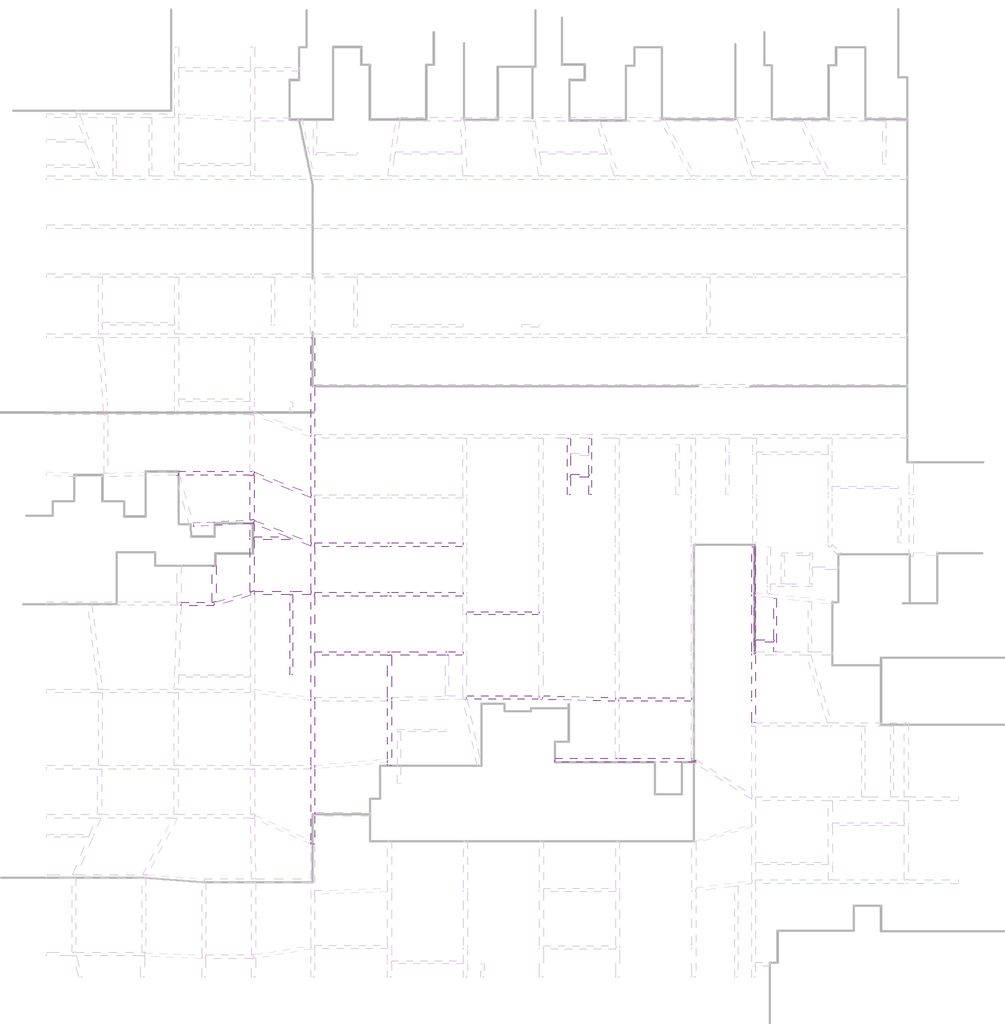
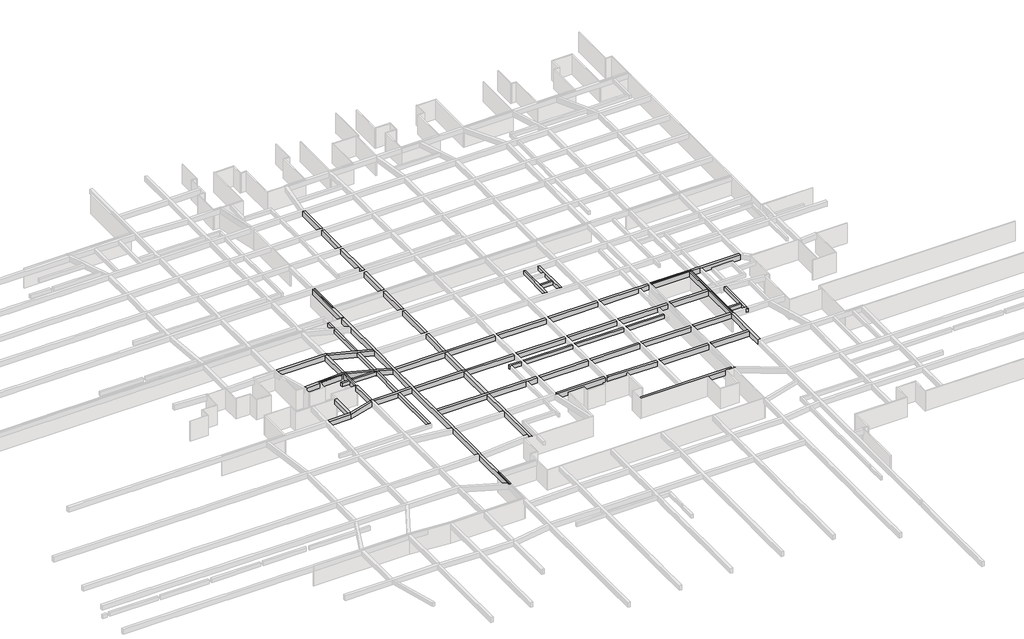
# One storey, part 13 of 16: 28 beams.
"""IFC4 building model written with IfcOpenShell, lengths in millimetres."""

from ifc_helpers import new_model, si_unit, frame, origin, place, context, project, spatial, polyline, outline, extrude, faceted_brep, element, save

model = new_model("IFC4")

# Units and contexts
model_context = context("Model", 3, world=origin())
ifc_project = project(units=[si_unit("LENGTHUNIT", "METRE", prefix="MILLI")], contexts=[model_context])

# Site, building, storey
site = spatial("IfcSite", under=ifc_project)
building = spatial("IfcBuilding", under=site)
storey = spatial("IfcBuildingStorey", under=building, Name="户型图", Elevation=0.0)

# Beams
placement = place(None, origin())
element("IfcBeam", 1, ObjectType="混凝土 - 矩形梁 : KL_beam", at=placement, inside=storey, context=model_context, shape_type="Brep", body=[
    faceted_brep([(127216.2109037, 158915.0633975, 3300.0), (127216.2109037, 158520.1276342, 3300.0), (127018.7754912, 158515.0633975, 3300.0), (127281.619868, 158515.0633975, 3300.0), (134828.9386535, 158515.0633975, 3300.0), (135228.9386535, 158515.0633975, 3300.0), (135228.9386535, 158852.5195892, 3300.0), (135228.9386535, 158915.0633975, 3300.0), (134828.9386535, 158915.0633975, 3300.0), (127018.7754912, 158515.0633975, 2500.0), (127281.619868, 158515.0633975, 2500.0), (134828.9386535, 158515.0633975, 2500.0), (135228.9386535, 158515.0633975, 2500.0), (127216.2109037, 158520.1276342, 2500.0), (127216.2109037, 158915.0633975, 2500.0), (134828.9386535, 158915.0633975, 2500.0), (135228.9386535, 158915.0633975, 2500.0), (135228.9386535, 158852.5195892, 2500.0)], [[[0, 1, 2, 3, 4, 5, 6, 7, 8]], [[2, 9, 10, 11, 12, 5, 4, 3]], [[13, 14, 15, 16, 17, 12, 11, 10, 9]], [[14, 0, 8, 7, 16, 15]], [[13, 1, 0, 14]], [[1, 13, 9, 2]], [[7, 6, 5, 12, 17, 16]]]),
])
element("IfcBeam", 2, ObjectType="混凝土 - 矩形梁 : KL_beam", at=placement, inside=storey, context=model_context, shape_type="Brep", body=[
    faceted_brep([(135228.9386535, 153383.6684969, 3300.0), (135228.9386535, 153710.917602, 3300.0), (135228.9386535, 153784.2174353, 3300.0), (134828.9386535, 153763.2543236, 3300.0), (128735.7458004, 153443.9236175, 3300.0), (128848.9009007, 153049.3048866, 3300.0), (134828.9386535, 153362.7053852, 3300.0), (134996.9527927, 153371.5106331, 3300.0), (135228.9386535, 153383.6684969, 2500.0), (128848.9009007, 153049.3048866, 2500.0), (134828.9386535, 153362.7053852, 2500.0), (134996.9527927, 153371.5106331, 2500.0), (135228.9386535, 153784.2174353, 2500.0), (135228.9386535, 153710.917602, 2500.0), (128735.7458004, 153443.9236175, 2500.0), (134828.9386535, 153763.2543236, 2500.0)], [[[0, 1, 2, 3, 4, 5, 6, 7]], [[8, 0, 7, 6, 5, 9, 10, 11]], [[12, 13, 8, 11, 10, 9, 14, 15]], [[2, 12, 15, 14, 4, 3]], [[5, 4, 14, 9]], [[2, 1, 0, 8, 13, 12]]]),
])
element("IfcBeam", 3, ObjectType="混凝土 - 矩形梁 : KL_beam", at=placement, inside=storey, context=model_context, shape_type="Brep", body=[
    faceted_brep([(135228.9386535, 158515.0633975, 3300.0), (134828.9386535, 158515.0633975, 3300.0), (134828.9386535, 153763.2543236, 3300.0), (135228.9386535, 153784.2174353, 3300.0), (135228.9386535, 158424.0615917, 3300.0), (134828.9386535, 158515.0633975, 2500.0), (134828.9386535, 153763.2543236, 2500.0), (135228.9386535, 158515.0633975, 2500.0), (135228.9386535, 158424.0615917, 2500.0), (135228.9386535, 153784.2174353, 2500.0)], [[[0, 1, 2, 3, 4]], [[1, 5, 6, 2]], [[5, 7, 8, 9, 6]], [[7, 0, 4, 3, 9, 8]], [[1, 0, 7, 5]], [[3, 2, 6, 9]]]),
])
element("IfcBeam", 4, ObjectType="混凝土 - 矩形梁 : KL_beam", at=placement, inside=storey, context=model_context, shape_type="Brep", body=[
    faceted_brep([(135228.9386535, 158852.5195892, 3300.0), (135228.9386535, 158515.0633975, 3300.0), (135228.9386535, 158424.0615917, 3300.0), (139049.0511844, 156957.6577813, 3300.0), (139349.0511844, 156842.4985708, 3300.0), (141266.2091209, 156106.5705895, 3300.0), (141266.2091209, 156535.028587, 3300.0), (139349.0511844, 157270.9565683, 3300.0), (139049.0511844, 157386.1157788, 3300.0), (135228.9386535, 158424.0615917, 2500.0), (141266.2091209, 156106.5705895, 2500.0), (135228.9386535, 158515.0633975, 2500.0), (135228.9386535, 158852.5195892, 2500.0), (141266.2091209, 156535.028587, 2500.0)], [[[0, 1, 2, 3, 4, 5, 6, 7, 8]], [[2, 9, 10, 5, 4, 3]], [[9, 11, 12, 13, 10]], [[12, 0, 8, 7, 6, 13]], [[0, 12, 11, 9, 2, 1]], [[6, 5, 10, 13]]]),
])
element("IfcBeam", 5, ObjectType="混凝土 - 矩形梁 : KL_beam", at=placement, inside=storey, context=model_context, shape_type="Brep", body=[
    faceted_brep([(135228.9386535, 153383.6684969, 3300.0), (134996.9527927, 153371.5106331, 3300.0), (135228.9386535, 153282.4596045, 3300.0), (138736.4375479, 151936.056926, 3300.0), (139049.0511844, 151816.0557941, 3300.0), (139349.0511844, 151700.8965836, 3300.0), (139517.9642674, 151636.056926, 3300.0), (141266.2091209, 150964.9686023, 3300.0), (141266.2091209, 151393.4265998, 3300.0), (139349.0511844, 152129.3545811, 3300.0), (139049.0511844, 152244.5137916, 3300.0), (135228.9386535, 153710.917602, 3300.0), (134996.9527927, 153371.5106331, 2500.0), (135228.9386535, 153282.4596045, 2500.0), (141266.2091209, 150964.9686023, 2500.0), (135228.9386535, 153383.6684969, 2500.0), (135228.9386535, 153710.917602, 2500.0), (141266.2091209, 151393.4265998, 2500.0)], [[[0, 1, 2, 3, 4, 5, 6, 7, 8, 9, 10, 11]], [[1, 12, 13, 14, 7, 6, 5, 4, 3, 2]], [[12, 15, 16, 17, 14, 13]], [[16, 11, 10, 9, 8, 17]], [[0, 15, 12, 1]], [[15, 0, 11, 16]], [[8, 7, 14, 17]]]),
])
element("IfcBeam", 6, ObjectType="混凝土 - 矩形梁 : KL_beam", at=placement, inside=storey, context=model_context, shape_type="Brep", body=[
    faceted_brep([(141266.2091209, 119283.141064, 3300.0), (141666.2091209, 119283.141064, 3300.0), (141666.2091209, 122278.0259701, 3300.0), (141666.2091209, 122678.0259701, 3300.0), (141666.2091209, 127294.7597353, 3300.0), (141666.2091209, 127696.2876703, 3300.0), (141666.2091209, 134512.5884701, 3300.0), (141666.2091209, 134912.5884701, 3300.0), (141666.2091209, 139362.5884701, 3300.0), (141666.2091209, 139762.5884701, 3300.0), (141666.2091209, 145662.5884701, 3300.0), (141666.2091209, 146062.5884701, 3300.0), (141666.2091209, 150902.424794, 3300.0), (141666.2091209, 151302.424794, 3300.0), (141666.2091209, 156044.0267812, 3300.0), (141666.2091209, 156444.0267812, 3300.0), (141666.2091209, 162447.0169772, 3300.0), (141666.2091209, 162847.0169772, 3300.0), (141666.2091209, 167762.578939, 3300.0), (141666.2091209, 168162.578939, 3300.0), (141666.2091209, 173112.5884701, 3300.0), (141266.2091209, 173112.5884701, 3300.0), (141266.2091209, 162932.5536596, 3300.0), (141266.2091209, 162504.0956621, 3300.0), (141266.2091209, 156535.028587, 3300.0), (141266.2091209, 156106.5705895, 3300.0), (141266.2091209, 151393.4265998, 3300.0), (141266.2091209, 150964.9686023, 3300.0), (141266.2091209, 146196.5023677, 3300.0), (141266.2091209, 145796.5023677, 3300.0), (141266.2091209, 134941.3479482, 3300.0), (141266.2091209, 134537.7323272, 3300.0), (141266.2091209, 127693.5189202, 3300.0), (141266.2091209, 127293.5189202, 3300.0), (141266.2091209, 119721.5942757, 3300.0), (141266.2091209, 119283.141064, 2500.0), (141266.2091209, 173112.5884701, 2500.0), (141266.2091209, 162932.5536596, 2500.0), (141266.2091209, 162504.0956621, 2500.0), (141266.2091209, 156535.028587, 2500.0), (141266.2091209, 156106.5705895, 2500.0), (141266.2091209, 151393.4265998, 2500.0), (141266.2091209, 150964.9686023, 2500.0), (141266.2091209, 146196.5023677, 2500.0), (141266.2091209, 145796.5023677, 2500.0), (141266.2091209, 134941.3479482, 2500.0), (141266.2091209, 134537.7323272, 2500.0), (141266.2091209, 127693.5189202, 2500.0), (141266.2091209, 127293.5189202, 2500.0), (141266.2091209, 119721.5942757, 2500.0), (141666.2091209, 119283.141064, 2500.0), (141666.2091209, 173112.5884701, 2500.0), (141666.2091209, 168162.578939, 2500.0), (141666.2091209, 167762.578939, 2500.0), (141666.2091209, 162847.0169772, 2500.0), (141666.2091209, 162447.0169772, 2500.0), (141666.2091209, 156444.0267812, 2500.0), (141666.2091209, 156044.0267812, 2500.0), (141666.2091209, 151302.424794, 2500.0), (141666.2091209, 150902.424794, 2500.0), (141666.2091209, 146062.5884701, 2500.0), (141666.2091209, 145662.5884701, 2500.0), (141666.2091209, 139762.5884701, 2500.0), (141666.2091209, 139362.5884701, 2500.0), (141666.2091209, 134912.5884701, 2500.0), (141666.2091209, 134512.5884701, 2500.0), (141666.2091209, 127696.2876703, 2500.0), (141666.2091209, 127294.7597353, 2500.0), (141666.2091209, 122678.0259701, 2500.0), (141666.2091209, 122278.0259701, 2500.0)], [[[0, 1, 2, 3, 4, 5, 6, 7, 8, 9, 10, 11, 12, 13, 14, 15, 16, 17, 18, 19, 20, 21, 22, 23, 24, 25, 26, 27, 28, 29, 30, 31, 32, 33, 34]], [[35, 0, 34, 33, 32, 31, 30, 29, 28, 27, 26, 25, 24, 23, 22, 21, 36, 37, 38, 39, 40, 41, 42, 43, 44, 45, 46, 47, 48, 49]], [[50, 35, 49, 48, 47, 46, 45, 44, 43, 42, 41, 40, 39, 38, 37, 36, 51, 52, 53, 54, 55, 56, 57, 58, 59, 60, 61, 62, 63, 64, 65, 66, 67, 68, 69]], [[1, 50, 69, 68, 67, 66, 65, 64, 63, 62, 61, 60, 59, 58, 57, 56, 55, 54, 53, 52, 51, 20, 19, 18, 17, 16, 15, 14, 13, 12, 11, 10, 9, 8, 7, 6, 5, 4, 3, 2]], [[21, 20, 51, 36]], [[1, 0, 35, 50]]]),
])
element("IfcBeam", 7, ObjectType="混凝土 - 矩形梁 : KL_beam", at=placement, inside=storey, context=model_context, shape_type="Brep", body=[
    faceted_brep([(141666.2091209, 151302.424794, 3300.0), (141666.2091209, 150902.424794, 3300.0), (149416.2109037, 150902.424794, 3300.0), (149816.2109037, 150902.424794, 3300.0), (157416.2109037, 150902.424794, 3300.0), (157416.2109037, 151302.424794, 3300.0), (149816.2109037, 151302.424794, 3300.0), (149416.2109037, 151302.424794, 3300.0), (141666.2091209, 150902.424794, 2500.0), (149416.2109037, 150902.424794, 2500.0), (149816.2109037, 150902.424794, 2500.0), (157416.2109037, 150902.424794, 2500.0), (141666.2091209, 151302.424794, 2500.0), (149416.2109037, 151302.424794, 2500.0), (149816.2109037, 151302.424794, 2500.0), (157416.2109037, 151302.424794, 2500.0)], [[[0, 1, 2, 3, 4, 5, 6, 7]], [[1, 8, 9, 10, 11, 4, 3, 2]], [[8, 12, 13, 14, 15, 11, 10, 9]], [[12, 0, 7, 6, 5, 15, 14, 13]], [[1, 0, 12, 8]], [[5, 4, 11, 15]]]),
    faceted_brep([(196226.5590225, 151302.424794, 3300.0), (196226.5590225, 150902.424794, 3300.0), (196226.5590225, 150902.424794, 2500.0), (196226.5590225, 151302.424794, 2500.0), (190074.1000448, 151302.424794, 3300.0), (189774.1000448, 151302.424794, 3300.0), (188616.2109037, 151302.424794, 3300.0), (188216.2109037, 151302.424794, 3300.0), (182116.2109037, 151302.424794, 3300.0), (182116.2109037, 151172.5884701, 3300.0), (188356.2109037, 151172.5884701, 3300.0), (188476.2109037, 151172.5884701, 3300.0), (188476.2109037, 150902.424794, 3300.0), (188516.2109037, 150902.424794, 3300.0), (189774.1000448, 150902.424794, 3300.0), (190074.1000448, 150902.424794, 3300.0), (188616.2109037, 151302.424794, 2500.0), (188216.2109037, 151302.424794, 2500.0), (182116.2109037, 151302.424794, 2500.0), (182116.2109037, 151172.5884701, 2500.0), (188476.2109037, 151172.5884701, 2500.0), (188476.2109037, 150902.424794, 2500.0), (188516.2109037, 150902.424794, 2500.0)], [[[0, 1, 2, 3]], [[1, 0, 4, 5, 6, 7, 8, 9, 10, 11, 12, 13, 14, 15]], [[0, 3, 16, 17, 18, 8, 7, 6, 5, 4]], [[8, 18, 19, 9]], [[12, 11, 20, 21]], [[2, 1, 15, 14, 13, 12, 21, 22]], [[20, 11, 10, 9, 19]], [[3, 2, 22, 21, 20, 19, 18, 17, 16]]]),
    faceted_brep([(157816.2109037, 150902.424794, 3300.0), (157816.2109037, 151302.424794, 3300.0), (157816.2109037, 151302.424794, 2500.0), (157816.2109037, 150902.424794, 2500.0), (165516.2109037, 151302.424794, 3300.0), (165516.2109037, 150902.424794, 3300.0), (165516.2109037, 150902.424794, 2500.0), (165516.2109037, 151302.424794, 2500.0)], [[[0, 1, 2, 3]], [[4, 5, 6, 7]], [[1, 0, 5, 4]], [[0, 3, 6, 5]], [[3, 2, 7, 6]], [[2, 1, 4, 7]]]),
    faceted_brep([(165916.2109037, 151302.424794, 3300.0), (165916.2109037, 150902.424794, 3300.0), (173616.2109037, 150902.424794, 3300.0), (173616.2109037, 151302.424794, 3300.0), (165916.2109037, 150902.424794, 2500.0), (173616.2109037, 150902.424794, 2500.0), (165916.2109037, 151302.424794, 2500.0), (173616.2109037, 151302.424794, 2500.0)], [[[0, 1, 2, 3]], [[1, 4, 5, 2]], [[4, 6, 7, 5]], [[6, 0, 3, 7]], [[1, 0, 6, 4]], [[3, 2, 5, 7]]]),
    faceted_brep([(174016.2109037, 150902.424794, 3300.0), (174016.2109037, 151302.424794, 3300.0), (174016.2109037, 151302.424794, 2500.0), (174016.2109037, 150902.424794, 2500.0), (181716.2109037, 151302.424794, 3300.0), (181716.2109037, 150902.424794, 3300.0), (181716.2109037, 150902.424794, 2500.0), (181716.2109037, 151302.424794, 2500.0), (180041.8640388, 150902.424794, 3300.0), (180341.8640388, 150902.424794, 3300.0), (180341.8640388, 151302.424794, 3300.0), (180041.8640388, 151302.424794, 3300.0)], [[[0, 1, 2, 3]], [[4, 5, 6, 7]], [[1, 0, 8, 9, 5, 4, 10, 11]], [[0, 3, 6, 5, 9, 8]], [[3, 2, 7, 6]], [[2, 1, 11, 10, 4, 7]]]),
    faceted_brep([(182116.2109037, 150902.424794, 3300.0), (182116.2109037, 150902.424794, 2500.0), (188116.2109037, 150902.424794, 2500.0), (188356.2109037, 150902.424794, 2500.0), (188356.2109037, 150902.424794, 3300.0), (188116.2109037, 150902.424794, 3300.0), (182116.2109037, 151052.5884701, 2500.0), (188356.2109037, 151052.5884701, 2500.0), (188356.2109037, 151052.5884701, 3300.0), (182116.2109037, 151052.5884701, 3300.0)], [[[0, 1, 2, 3, 4, 5]], [[3, 2, 1, 6, 7]], [[4, 3, 7, 8]], [[9, 8, 7, 6]], [[0, 5, 4, 8, 9]], [[1, 0, 9, 6]]]),
])
element("IfcBeam", 8, ObjectType="混凝土 - 矩形梁 : KL_beam", at=placement, inside=storey, context=model_context, shape_type="Brep", body=[
    faceted_brep([(141666.2091209, 146062.5884701, 3300.0), (141666.2091209, 145662.5884701, 3300.0), (149416.2109037, 145662.5884701, 3300.0), (149816.2109037, 145662.5884701, 3300.0), (157416.2109037, 145662.5884701, 3300.0), (157416.2109037, 146062.5884701, 3300.0), (149816.2109037, 146062.5884701, 3300.0), (149416.2109037, 146062.5884701, 3300.0), (141666.2091209, 145662.5884701, 2500.0), (149416.2109037, 145662.5884701, 2500.0), (149816.2109037, 145662.5884701, 2500.0), (157416.2109037, 145662.5884701, 2500.0), (141666.2091209, 146062.5884701, 2500.0), (149416.2109037, 146062.5884701, 2500.0), (149816.2109037, 146062.5884701, 2500.0), (157416.2109037, 146062.5884701, 2500.0)], [[[0, 1, 2, 3, 4, 5, 6, 7]], [[1, 8, 9, 10, 11, 4, 3, 2]], [[8, 12, 13, 14, 15, 11, 10, 9]], [[12, 0, 7, 6, 5, 15, 14, 13]], [[1, 0, 12, 8]], [[5, 4, 11, 15]]]),
    faceted_brep([(157816.2109037, 145662.5884701, 3300.0), (157816.2109037, 146062.5884701, 3300.0), (157816.2109037, 146062.5884701, 2500.0), (157816.2109037, 145662.5884701, 2500.0), (165516.2109037, 146062.5884701, 3300.0), (165516.2109037, 145662.5884701, 3300.0), (165516.2109037, 145662.5884701, 2500.0), (165516.2109037, 146062.5884701, 2500.0)], [[[0, 1, 2, 3]], [[4, 5, 6, 7]], [[1, 0, 5, 4]], [[0, 3, 6, 5]], [[3, 2, 7, 6]], [[2, 1, 4, 7]]]),
    faceted_brep([(165916.2109037, 146062.5884701, 3300.0), (165916.2109037, 145662.5884701, 3300.0), (173616.2109037, 145662.5884701, 3300.0), (173616.2109037, 146062.5884701, 3300.0), (165916.2109037, 145662.5884701, 2500.0), (173616.2109037, 145662.5884701, 2500.0), (165916.2109037, 146062.5884701, 2500.0), (173616.2109037, 146062.5884701, 2500.0)], [[[0, 1, 2, 3]], [[1, 4, 5, 2]], [[4, 6, 7, 5]], [[6, 0, 3, 7]], [[1, 0, 6, 4]], [[3, 2, 5, 7]]]),
    faceted_brep([(174016.2109037, 145662.5884701, 3300.0), (174016.2109037, 146062.5884701, 3300.0), (174016.2109037, 146062.5884701, 2500.0), (174016.2109037, 145662.5884701, 2500.0), (181716.2109037, 146062.5884701, 3300.0), (181716.2109037, 145662.5884701, 3300.0), (181716.2109037, 145662.5884701, 2500.0), (181716.2109037, 146062.5884701, 2500.0), (180041.8640388, 145662.5884701, 3300.0), (180341.8640388, 145662.5884701, 3300.0), (180341.8640388, 146062.5884701, 3300.0), (180041.8640388, 146062.5884701, 3300.0)], [[[0, 1, 2, 3]], [[4, 5, 6, 7]], [[1, 0, 8, 9, 5, 4, 10, 11]], [[0, 3, 6, 5, 9, 8]], [[3, 2, 7, 6]], [[2, 1, 11, 10, 4, 7]]]),
    faceted_brep([(182116.2109037, 145662.5884701, 3300.0), (182116.2109037, 146062.5884701, 3300.0), (182116.2109037, 146062.5884701, 2500.0), (182116.2109037, 145662.5884701, 2500.0), (188116.2109037, 145662.5884701, 3300.0), (188116.2109037, 146062.5884701, 3300.0), (188116.2109037, 145662.5884701, 2500.0), (188116.2109037, 146062.5884701, 2500.0)], [[[0, 1, 2, 3]], [[1, 0, 4, 5]], [[0, 3, 6, 4]], [[3, 2, 7, 6]], [[2, 1, 5, 7]], [[5, 4, 6, 7]]]),
])
element("IfcBeam", 9, ObjectType="混凝土 - 矩形梁 : KL_beam", at=placement, inside=storey, context=model_context, shape_type="Brep", body=[
    faceted_brep([(141666.2091209, 139762.5884701, 3300.0), (141666.2091209, 139362.5884701, 3300.0), (149416.2109037, 139362.5884701, 3300.0), (149816.2109037, 139362.5884701, 3300.0), (155575.8505966, 139362.5884701, 3300.0), (155875.8505966, 139362.5884701, 3300.0), (157416.2109037, 139362.5884701, 3300.0), (157416.2109037, 139762.5884701, 3300.0), (155875.8505966, 139762.5884701, 3300.0), (155575.8505966, 139762.5884701, 3300.0), (149816.2109037, 139762.5884701, 3300.0), (149416.2109037, 139762.5884701, 3300.0), (141666.2091209, 139362.5884701, 2500.0), (149416.2109037, 139362.5884701, 2500.0), (149816.2109037, 139362.5884701, 2500.0), (157416.2109037, 139362.5884701, 2500.0), (141666.2091209, 139762.5884701, 2500.0), (149416.2109037, 139762.5884701, 2500.0), (149816.2109037, 139762.5884701, 2500.0), (157416.2109037, 139762.5884701, 2500.0)], [[[0, 1, 2, 3, 4, 5, 6, 7, 8, 9, 10, 11]], [[1, 12, 13, 14, 15, 6, 5, 4, 3, 2]], [[12, 16, 17, 18, 19, 15, 14, 13]], [[16, 0, 11, 10, 9, 8, 7, 19, 18, 17]], [[1, 0, 16, 12]], [[7, 6, 15, 19]]]),
    faceted_brep([(157816.2109037, 139362.5884701, 3300.0), (157816.2109037, 139762.5884701, 3300.0), (157816.2109037, 139762.5884701, 2500.0), (157816.2109037, 139362.5884701, 2500.0), (165516.2109037, 139762.5884701, 3300.0), (165516.2109037, 139362.5884701, 3300.0), (165516.2109037, 139362.5884701, 2500.0), (165516.2109037, 139762.5884701, 2500.0)], [[[0, 1, 2, 3]], [[4, 5, 6, 7]], [[1, 0, 5, 4]], [[0, 3, 6, 5]], [[3, 2, 7, 6]], [[2, 1, 4, 7]]]),
    faceted_brep([(165916.2109037, 139762.5884701, 3300.0), (165916.2109037, 139362.5884701, 3300.0), (173616.2109037, 139362.5884701, 3300.0), (173616.2109037, 139762.5884701, 3300.0), (165916.2109037, 139362.5884701, 2500.0), (173616.2109037, 139362.5884701, 2500.0), (165916.2109037, 139762.5884701, 2500.0), (173616.2109037, 139762.5884701, 2500.0)], [[[0, 1, 2, 3]], [[1, 4, 5, 2]], [[4, 6, 7, 5]], [[6, 0, 3, 7]], [[1, 0, 6, 4]], [[3, 2, 5, 7]]]),
    faceted_brep([(174016.2109037, 139362.5884701, 3300.0), (174016.2109037, 139762.5884701, 3300.0), (174016.2109037, 139762.5884701, 2500.0), (174016.2109037, 139362.5884701, 2500.0), (181716.2109037, 139762.5884701, 3300.0), (181716.2109037, 139362.5884701, 3300.0), (181716.2109037, 139362.5884701, 2500.0), (181716.2109037, 139762.5884701, 2500.0)], [[[0, 1, 2, 3]], [[4, 5, 6, 7]], [[1, 0, 5, 4]], [[0, 3, 6, 5]], [[3, 2, 7, 6]], [[2, 1, 4, 7]]]),
    faceted_brep([(182116.2109037, 139362.5884701, 3300.0), (182116.2109037, 139762.5884701, 3300.0), (182116.2109037, 139762.5884701, 2500.0), (182116.2109037, 139362.5884701, 2500.0), (188116.2109037, 139362.5884701, 3300.0), (188116.2109037, 139762.5884701, 3300.0), (188116.2109037, 139362.5884701, 2500.0), (188116.2109037, 139762.5884701, 2500.0)], [[[0, 1, 2, 3]], [[1, 0, 4, 5]], [[0, 3, 6, 4]], [[3, 2, 7, 6]], [[2, 1, 5, 7]], [[5, 4, 6, 7]]]),
])
element("IfcBeam", 10, ObjectType="混凝土 - 矩形梁 : KL_beam", at=placement, inside=storey, context=model_context, shape_type="Brep", body=[
    faceted_brep([(157816.2109037, 135095.7397162, 3300.0), (157816.2109037, 134700.2382994, 3300.0), (157618.4857796, 134695.7397162, 3300.0), (157863.190335, 134695.7397162, 3300.0), (165516.2109037, 134695.7397162, 3300.0), (165516.2109037, 135095.7397162, 3300.0), (157618.4857796, 134695.7397162, 2500.0), (157863.190335, 134695.7397162, 2500.0), (165516.2109037, 134695.7397162, 2500.0), (157816.2109037, 134700.2382994, 2500.0), (157816.2109037, 135095.7397162, 2500.0), (165516.2109037, 135095.7397162, 2500.0)], [[[0, 1, 2, 3, 4, 5]], [[2, 6, 7, 8, 4, 3]], [[9, 10, 11, 8, 7, 6]], [[10, 0, 5, 11]], [[9, 1, 0, 10]], [[1, 9, 6, 2]], [[5, 4, 8, 11]]]),
])
element("IfcBeam", 11, ObjectType="混凝土 - 矩形梁 : KL_beam", at=placement, inside=storey, context=model_context, shape_type="SweptSolid", body=[
    extrude(outline(polyline([(165916.2109037, 134695.7397162), (165916.2109037, 135090.2366531), (173616.2109037, 134875.3714487), (173616.2109037, 134475.2157459), (165713.4209895, 134695.7397162), (165916.2109037, 134695.7397162)])), frame((0.0, 0.0, 2500.0), z_axis=(0.0, 0.0, 1.0), x_axis=(1.0, 0.0, 0.0)), (0.0, 0.0, 1.0), 800.0),
])
element("IfcBeam", 12, ObjectType="混凝土 - 矩形梁 : KL_beam", at=placement, inside=storey, context=model_context, shape_type="SweptSolid", body=[
    extrude(outline(polyline([(174016.2109037, 134469.7126829), (174016.2109037, 134869.7126829), (181716.2109037, 134869.7126829), (181716.2109037, 134469.7126829), (174016.2109037, 134469.7126829)])), frame((0.0, 0.0, 2500.0), z_axis=(0.0, 0.0, 1.0), x_axis=(1.0, 0.0, 0.0)), (0.0, 0.0, 1.0), 800.0),
    extrude(outline(polyline([(182116.2109037, 134469.7126829), (182116.2109037, 134869.7126829), (188116.2109037, 134869.7126829), (188116.2109037, 134469.7126829), (182116.2109037, 134469.7126829)])), frame((0.0, 0.0, 2500.0), z_axis=(0.0, 0.0, 1.0), x_axis=(1.0, 0.0, 0.0)), (0.0, 0.0, 1.0), 800.0),
])
element("IfcBeam", 13, ObjectType="混凝土 - 矩形梁 : KL_beam", at=placement, inside=storey, context=model_context, shape_type="Brep", body=[
    faceted_brep([(167203.7499662, 128412.5884701, 3300.0), (167203.7499662, 128412.5884701, 2500.0), (167203.7499662, 128012.5884701, 2500.0), (167203.7499662, 128012.5884701, 3300.0), (182116.2109037, 128012.5884701, 3300.0), (182116.2109037, 128072.5884701, 3300.0), (182116.2109037, 128212.6640931, 3300.0), (182017.7367524, 128212.6640931, 3300.0), (182017.7367524, 128072.5884701, 3300.0), (181897.7367524, 128072.5884701, 3300.0), (181897.7367524, 128212.6640931, 3300.0), (181716.2109037, 128212.6640931, 3300.0), (181716.2109037, 128412.5884701, 3300.0), (174016.2109037, 128412.5884701, 3300.0), (173616.2109037, 128412.5884701, 3300.0), (182116.2109037, 128012.5884701, 2500.0), (173616.2109037, 128412.5884701, 2500.0), (174016.2109037, 128412.5884701, 2500.0), (181716.2109037, 128412.5884701, 2500.0), (181716.2109037, 128212.6640931, 2500.0), (181897.7367524, 128212.6640931, 2500.0), (181897.7367524, 128072.5884701, 2500.0), (182017.7367524, 128072.5884701, 2500.0), (182017.7367524, 128212.6640931, 2500.0), (182116.2109037, 128212.6640931, 2500.0), (182116.2109037, 128072.5884701, 2500.0)], [[[0, 1, 2, 3]], [[0, 3, 4, 5, 6, 7, 8, 9, 10, 11, 12, 13, 14]], [[3, 2, 15, 4]], [[2, 1, 16, 17, 18, 19, 20, 21, 22, 23, 24, 25, 15]], [[1, 0, 14, 13, 12, 18, 17, 16]], [[4, 15, 25, 24, 6, 5]], [[12, 11, 19, 18]], [[6, 24, 23, 7]], [[22, 8, 7, 23]], [[9, 21, 20, 10]], [[8, 22, 21, 9]], [[19, 11, 10, 20]]]),
])
element("IfcBeam", 14, ObjectType="混凝土 - 矩形梁 : KL_beam", at=placement, inside=storey, context=model_context, shape_type="Brep", body=[
    faceted_brep([(149816.2109037, 127638.3828431, 3300.0), (149416.2109037, 127638.3828431, 3300.0), (149416.2109037, 127638.3828431, 2500.0), (149816.2109037, 127638.3828431, 2500.0), (149816.2109037, 134518.224679, 3300.0), (149816.2109037, 134918.3281936, 3300.0), (149816.2109037, 139362.5884701, 3300.0), (149416.2109037, 139362.5884701, 3300.0), (149416.2109037, 134912.5884701, 3300.0), (149416.2109037, 134512.5884701, 3300.0), (149416.2109037, 128374.3249686, 3300.0), (149416.2109037, 127972.7970336, 3300.0), (149416.2109037, 139362.5884701, 2500.0), (149416.2109037, 134912.5884701, 2500.0), (149416.2109037, 134512.5884701, 2500.0), (149416.2109037, 128374.3249686, 2500.0), (149416.2109037, 127972.7970336, 2500.0), (149816.2109037, 139362.5884701, 2500.0), (149816.2109037, 134918.3281936, 2500.0), (149816.2109037, 134518.224679, 2500.0)], [[[0, 1, 2, 3]], [[1, 0, 4, 5, 6, 7, 8, 9, 10, 11]], [[2, 1, 11, 10, 9, 8, 7, 12, 13, 14, 15, 16]], [[3, 2, 16, 15, 14, 13, 12, 17, 18, 19]], [[0, 3, 19, 18, 17, 6, 5, 4]], [[7, 6, 17, 12]]]),
    faceted_brep([(149416.2109037, 189895.7397162, 3300.0), (149816.2109037, 189895.7397162, 3300.0), (149816.2109037, 189895.7397162, 2500.0), (149416.2109037, 189895.7397162, 2500.0), (149816.2109037, 185072.5884701, 3300.0), (149416.2109037, 185072.5884701, 3300.0), (149416.2109037, 185072.5884701, 2500.0), (149816.2109037, 185072.5884701, 2500.0)], [[[0, 1, 2, 3]], [[4, 5, 6, 7]], [[1, 0, 5, 4]], [[0, 3, 6, 5]], [[3, 2, 7, 6]], [[2, 1, 4, 7]]]),
    faceted_brep([(149416.2109037, 184672.5884701, 3300.0), (149816.2109037, 184672.5884701, 3300.0), (149816.2109037, 184672.5884701, 2500.0), (149416.2109037, 184672.5884701, 2500.0), (149816.2109037, 179912.5884701, 3300.0), (149416.2109037, 179912.5884701, 3300.0), (149416.2109037, 179912.5884701, 2500.0), (149816.2109037, 179912.5884701, 2500.0)], [[[0, 1, 2, 3]], [[4, 5, 6, 7]], [[1, 0, 5, 4]], [[0, 3, 6, 5]], [[3, 2, 7, 6]], [[2, 1, 4, 7]]]),
    faceted_brep([(149416.2109037, 179512.5884701, 3300.0), (149816.2109037, 179512.5884701, 3300.0), (149816.2109037, 179512.5884701, 2500.0), (149416.2109037, 179512.5884701, 2500.0), (149816.2109037, 173512.5884701, 3300.0), (149416.2109037, 173512.5884701, 3300.0), (149416.2109037, 173512.5884701, 2500.0), (149816.2109037, 173512.5884701, 2500.0), (149416.2109037, 174520.6993439, 3300.0), (149416.2109037, 174220.6993439, 3300.0), (149816.2109037, 174220.6993439, 3300.0), (149816.2109037, 174520.6993439, 3300.0)], [[[0, 1, 2, 3]], [[4, 5, 6, 7]], [[1, 0, 8, 9, 5, 4, 10, 11]], [[0, 3, 6, 5, 9, 8]], [[3, 2, 7, 6]], [[2, 1, 11, 10, 4, 7]]]),
    faceted_brep([(149416.2109037, 173112.5884701, 3300.0), (149816.2109037, 173112.5884701, 3300.0), (149816.2109037, 173112.5884701, 2500.0), (149416.2109037, 173112.5884701, 2500.0), (149816.2109037, 168162.578939, 3300.0), (149416.2109037, 168162.578939, 3300.0), (149416.2109037, 168162.578939, 2500.0), (149816.2109037, 168162.578939, 2500.0)], [[[0, 1, 2, 3]], [[4, 5, 6, 7]], [[1, 0, 5, 4]], [[0, 3, 6, 5]], [[3, 2, 7, 6]], [[2, 1, 4, 7]]]),
    faceted_brep([(149416.2109037, 162447.0169772, 3300.0), (149816.2109037, 162447.0169772, 3300.0), (149816.2109037, 162447.0169772, 2500.0), (149416.2109037, 162447.0169772, 2500.0), (149816.2109037, 156444.0267812, 3300.0), (149416.2109037, 156444.0267812, 3300.0), (149416.2109037, 156444.0267812, 2500.0), (149816.2109037, 156444.0267812, 2500.0)], [[[0, 1, 2, 3]], [[4, 5, 6, 7]], [[1, 0, 5, 4]], [[0, 3, 6, 5]], [[3, 2, 7, 6]], [[2, 1, 4, 7]]]),
    faceted_brep([(149816.2109037, 162847.0169772, 3300.0), (149416.2109037, 162847.0169772, 3300.0), (149416.2109037, 162847.0169772, 2500.0), (149816.2109037, 162847.0169772, 2500.0), (149816.2109037, 167762.578939, 3300.0), (149416.2109037, 167762.578939, 3300.0), (149416.2109037, 167762.578939, 2500.0), (149816.2109037, 167762.578939, 2500.0)], [[[0, 1, 2, 3]], [[1, 0, 4, 5]], [[2, 1, 5, 6]], [[3, 2, 6, 7]], [[0, 3, 7, 4]], [[5, 4, 7, 6]]]),
    faceted_brep([(149416.2109037, 156044.0267812, 3300.0), (149816.2109037, 156044.0267812, 3300.0), (149816.2109037, 156044.0267812, 2500.0), (149416.2109037, 156044.0267812, 2500.0), (149816.2109037, 151302.424794, 3300.0), (149416.2109037, 151302.424794, 3300.0), (149416.2109037, 151302.424794, 2500.0), (149816.2109037, 151302.424794, 2500.0)], [[[0, 1, 2, 3]], [[4, 5, 6, 7]], [[1, 0, 5, 4]], [[0, 3, 6, 5]], [[3, 2, 7, 6]], [[2, 1, 4, 7]]]),
    faceted_brep([(149416.2109037, 150902.424794, 3300.0), (149816.2109037, 150902.424794, 3300.0), (149816.2109037, 150902.424794, 2500.0), (149416.2109037, 150902.424794, 2500.0), (149816.2109037, 146062.5884701, 3300.0), (149416.2109037, 146062.5884701, 3300.0), (149416.2109037, 146062.5884701, 2500.0), (149816.2109037, 146062.5884701, 2500.0)], [[[0, 1, 2, 3]], [[4, 5, 6, 7]], [[1, 0, 5, 4]], [[0, 3, 6, 5]], [[3, 2, 7, 6]], [[2, 1, 4, 7]]]),
    faceted_brep([(149416.2109037, 145662.5884701, 3300.0), (149816.2109037, 145662.5884701, 3300.0), (149816.2109037, 145662.5884701, 2500.0), (149416.2109037, 145662.5884701, 2500.0), (149816.2109037, 139762.5884701, 3300.0), (149416.2109037, 139762.5884701, 3300.0), (149416.2109037, 139762.5884701, 2500.0), (149816.2109037, 139762.5884701, 2500.0)], [[[0, 1, 2, 3]], [[4, 5, 6, 7]], [[1, 0, 5, 4]], [[0, 3, 6, 5]], [[3, 2, 7, 6]], [[2, 1, 4, 7]]]),
])
element("IfcBeam", 15, ObjectType="混凝土 - 矩形梁 : KL_beam", at=placement, inside=storey, context=model_context, shape_type="Brep", body=[
    faceted_brep([(188116.2109037, 132211.3072201, 3300.0), (188516.2109037, 132211.3072201, 3300.0), (188516.2109037, 139362.5884701, 3300.0), (188516.2109037, 139762.5884701, 3300.0), (188516.2109037, 140731.0377403, 3300.0), (188516.2109037, 141031.0377403, 3300.0), (188516.2109037, 145641.0174941, 3300.0), (188516.2109037, 146043.11753, 3300.0), (188516.2109037, 146655.8638084, 3300.0), (188516.2109037, 146955.8638084, 3300.0), (188516.2109037, 150902.424794, 3300.0), (188476.2109037, 150902.424794, 3300.0), (188476.2109037, 139562.5884701, 3300.0), (188356.2109037, 139562.5884701, 3300.0), (188356.2109037, 150902.424794, 3300.0), (188116.2109037, 150902.424794, 3300.0), (188116.2109037, 146062.5884701, 3300.0), (188116.2109037, 145662.5884701, 3300.0), (188116.2109037, 139762.5884701, 3300.0), (188116.2109037, 139362.5884701, 3300.0), (188116.2109037, 134869.7126829, 3300.0), (188116.2109037, 134469.7126829, 3300.0), (188516.2109037, 132211.3072201, 2500.0), (188516.2109037, 139362.5884701, 2500.0), (188516.2109037, 139762.5884701, 2500.0), (188516.2109037, 145641.0174941, 2500.0), (188516.2109037, 146043.11753, 2500.0), (188516.2109037, 150902.424794, 2500.0), (188116.2109037, 132211.3072201, 2500.0), (188116.2109037, 134469.7126829, 2500.0), (188116.2109037, 134869.7126829, 2500.0), (188116.2109037, 139362.5884701, 2500.0), (188116.2109037, 139762.5884701, 2500.0), (188116.2109037, 145662.5884701, 2500.0), (188116.2109037, 146062.5884701, 2500.0), (188116.2109037, 150902.424794, 2500.0), (188356.2109037, 150902.424794, 2500.0), (188356.2109037, 139562.5884701, 2500.0), (188476.2109037, 139562.5884701, 2500.0), (188476.2109037, 150902.424794, 2500.0)], [[[0, 1, 2, 3, 4, 5, 6, 7, 8, 9, 10, 11, 12, 13, 14, 15, 16, 17, 18, 19, 20, 21]], [[1, 22, 23, 24, 25, 26, 27, 10, 9, 8, 7, 6, 5, 4, 3, 2]], [[22, 28, 29, 30, 31, 32, 33, 34, 35, 36, 37, 38, 39, 27, 26, 25, 24, 23]], [[28, 0, 21, 20, 19, 18, 17, 16, 15, 35, 34, 33, 32, 31, 30, 29]], [[1, 0, 28, 22]], [[35, 15, 14, 36]], [[13, 37, 36, 14]], [[38, 12, 11, 39]], [[10, 27, 39, 11]], [[37, 13, 12, 38]]]),
])
element("IfcBeam", 16, ObjectType="混凝土 - 矩形梁 : KL_beam", at=placement, inside=storey, context=model_context, shape_type="Brep", body=[
    faceted_brep([(131003.4020759, 144613.3955863, 3300.0), (130946.8040559, 145013.3955863, 3300.0), (130775.1030659, 145013.3955863, 3300.0), (127482.2091287, 145013.3955863, 3300.0), (127468.2408209, 144613.3955863, 3300.0), (131003.4020759, 144613.3955863, 2500.0), (127468.2408209, 144613.3955863, 2500.0), (130946.8040559, 145013.3955863, 2500.0), (127482.2091287, 145013.3955863, 2500.0), (130775.1030659, 145013.3955863, 2500.0)], [[[0, 1, 2, 3, 4]], [[5, 0, 4, 6]], [[7, 5, 6, 8, 9]], [[1, 7, 9, 8, 3, 2]], [[4, 3, 8, 6]], [[1, 0, 5, 7]]]),
])
element("IfcBeam", 17, ObjectType="混凝土 - 矩形梁 : KL_beam", at=placement, inside=storey, context=model_context, shape_type="Brep", body=[
    faceted_brep([(134872.1367776, 146146.9200065, 3300.0), (134869.7438693, 146146.2290026, 3300.0), (134828.9386535, 146134.4456171, 3300.0), (131175.1030659, 145079.3218456, 3300.0), (130946.8040559, 145013.3955863, 3300.0), (131003.4020759, 144613.3955863, 3300.0), (134872.1367776, 145730.5761084, 3300.0), (131003.4020759, 144613.3955863, 2500.0), (134872.1367776, 145730.5761084, 2500.0), (130946.8040559, 145013.3955863, 2500.0), (131175.1030659, 145079.3218456, 2500.0), (134828.9386535, 146134.4456171, 2500.0), (134869.7438693, 146146.2290026, 2500.0), (134872.1367776, 146146.9200065, 2500.0)], [[[0, 1, 2, 3, 4, 5, 6]], [[5, 7, 8, 6]], [[9, 10, 11, 12, 13, 8, 7]], [[4, 3, 2, 1, 0, 13, 12, 11, 10, 9]], [[4, 9, 7, 5]], [[0, 6, 8, 13]]]),
])
element("IfcBeam", 18, ObjectType="混凝土 - 矩形梁 : KL_beam", at=placement, inside=storey, context=model_context, shape_type="Brep", body=[
    faceted_brep([(134872.1367776, 146146.9200065, 3300.0), (135272.1367776, 146146.9200065, 3300.0), (135272.1367776, 145846.084729, 3300.0), (135272.1367776, 145796.5023677, 3300.0), (139049.0511844, 145796.5023677, 3300.0), (139349.0511844, 145796.5023677, 3300.0), (141266.2091209, 145796.5023677, 3300.0), (141266.2091209, 146196.5023677, 3300.0), (139349.0511844, 146196.5023677, 3300.0), (139049.0511844, 146196.5023677, 3300.0), (135228.9386535, 146196.5023677, 3300.0), (134869.7438693, 146196.5023677, 3300.0), (134869.7438693, 146146.2290026, 3300.0), (135272.1367776, 145796.5023677, 2500.0), (141266.2091209, 145796.5023677, 2500.0), (135272.1367776, 146146.9200065, 2500.0), (134872.1367776, 146146.9200065, 2500.0), (134869.7438693, 146146.2290026, 2500.0), (134869.7438693, 146196.5023677, 2500.0), (135228.9386535, 146196.5023677, 2500.0), (141266.2091209, 146196.5023677, 2500.0), (135272.1367776, 145846.084729, 2500.0)], [[[0, 1, 2, 3, 4, 5, 6, 7, 8, 9, 10, 11, 12]], [[3, 13, 14, 6, 5, 4]], [[15, 16, 17, 18, 19, 20, 14, 13, 21]], [[18, 11, 10, 9, 8, 7, 20, 19]], [[11, 18, 17, 12]], [[1, 15, 21, 13, 3, 2]], [[15, 1, 0, 16]], [[16, 0, 12, 17]], [[7, 6, 14, 20]]]),
])
element("IfcBeam", 19, ObjectType="混凝土 - 矩形梁 : KL_beam", at=placement, inside=storey, context=model_context, shape_type="Brep", body=[
    faceted_brep([(134996.9527927, 153371.5106331, 3300.0), (134828.9386535, 153362.7053852, 3300.0), (134828.9386535, 151936.056926, 3300.0), (134828.9386535, 151636.056926, 3300.0), (134828.9386535, 146134.4456171, 3300.0), (134869.7438693, 146146.2290026, 3300.0), (134869.7438693, 146196.5023677, 3300.0), (135228.9386535, 146196.5023677, 3300.0), (135228.9386535, 151636.056926, 3300.0), (135228.9386535, 151936.056926, 3300.0), (135228.9386535, 153282.4596045, 3300.0), (134828.9386535, 153362.7053852, 2500.0), (134828.9386535, 146134.4456171, 2500.0), (134996.9527927, 153371.5106331, 2500.0), (135228.9386535, 153282.4596045, 2500.0), (135228.9386535, 146196.5023677, 2500.0), (134869.7438693, 146196.5023677, 2500.0), (134869.7438693, 146146.2290026, 2500.0)], [[[0, 1, 2, 3, 4, 5, 6, 7, 8, 9, 10]], [[1, 11, 12, 4, 3, 2]], [[11, 13, 14, 15, 16, 17, 12]], [[14, 10, 9, 8, 7, 15]], [[11, 1, 0, 13]], [[0, 10, 14, 13]], [[4, 12, 17, 5]], [[6, 16, 15, 7]], [[16, 6, 5, 17]]]),
])
element("IfcBeam", 20, ObjectType="混凝土 - 矩形梁 : KL_beam", at=placement, inside=storey, context=model_context, shape_type="SweptSolid", body=[
    extrude(outline(polyline([(130775.1030659, 148884.5232782), (131175.1030659, 148884.5232782), (131175.1030659, 145079.3218456), (130946.8040559, 145013.3955863), (130775.1030659, 145013.3955863), (130775.1030659, 148884.5232782)])), frame((0.0, 0.0, 2500.0), z_axis=(0.0, 0.0, 1.0), x_axis=(1.0, 0.0, 0.0)), (0.0, 0.0, 1.0), 800.0),
])
element("IfcBeam", 21, ObjectType="混凝土 - 矩形梁 : L_beam", at=placement, inside=storey, context=model_context, shape_type="Brep", body=[
    faceted_brep([(168841.2109037, 162447.0169772, 3300.0), (168541.2109037, 162447.0169772, 3300.0), (168541.2109037, 156444.0267812, 3300.0), (168841.2109037, 156444.0267812, 3300.0), (168841.2109037, 158287.5884701, 3300.0), (168841.2109037, 158587.5884701, 3300.0), (168841.2109037, 160537.5884701, 3300.0), (168841.2109037, 160837.5884701, 3300.0), (168541.2109037, 162447.0169772, 2700.0), (168541.2109037, 156444.0267812, 2700.0), (168841.2109037, 162447.0169772, 2700.0), (168841.2109037, 160837.5884701, 2700.0), (168841.2109037, 160537.5884701, 2700.0), (168841.2109037, 158587.5884701, 2700.0), (168841.2109037, 158287.5884701, 2700.0), (168841.2109037, 156444.0267812, 2700.0)], [[[0, 1, 2, 3, 4, 5, 6, 7]], [[1, 8, 9, 2]], [[8, 10, 11, 12, 13, 14, 15, 9]], [[10, 0, 7, 6, 5, 4, 3, 15, 14, 13, 12, 11]], [[1, 0, 10, 8]], [[3, 2, 9, 15]]]),
])
element("IfcBeam", 22, ObjectType="混凝土 - 矩形梁 : L_beam", at=placement, inside=storey, context=model_context, shape_type="Brep", body=[
    faceted_brep([(171091.2109037, 162447.0169772, 3300.0), (170791.2109037, 162447.0169772, 3300.0), (170791.2109037, 160837.5884701, 3300.0), (170791.2109037, 160537.5884701, 3300.0), (170791.2109037, 158587.5884701, 3300.0), (170791.2109037, 158287.5884701, 3300.0), (170791.2109037, 156444.0267812, 3300.0), (171091.2109037, 156444.0267812, 3300.0), (170791.2109037, 162447.0169772, 2700.0), (170791.2109037, 160837.5884701, 2700.0), (170791.2109037, 160537.5884701, 2700.0), (170791.2109037, 158587.5884701, 2700.0), (170791.2109037, 158287.5884701, 2700.0), (170791.2109037, 156444.0267812, 2700.0), (171091.2109037, 162447.0169772, 2700.0), (171091.2109037, 156444.0267812, 2700.0)], [[[0, 1, 2, 3, 4, 5, 6, 7]], [[1, 8, 9, 10, 11, 12, 13, 6, 5, 4, 3, 2]], [[8, 14, 15, 13, 12, 11, 10, 9]], [[14, 0, 7, 15]], [[1, 0, 14, 8]], [[7, 6, 13, 15]]]),
])
element("IfcBeam", 23, ObjectType="混凝土 - 矩形梁 : L_beam", at=placement, inside=storey, context=model_context, shape_type="SweptSolid", body=[
    extrude(outline(polyline([(168841.2109037, 158287.5884701), (168841.2109037, 158587.5884701), (170791.2109037, 158587.5884701), (170791.2109037, 158287.5884701), (168841.2109037, 158287.5884701)])), frame((0.0, 0.0, 2700.0), z_axis=(0.0, 0.0, 1.0), x_axis=(1.0, 0.0, 0.0)), (0.0, 0.0, 1.0), 600.0),
])
element("IfcBeam", 24, ObjectType="混凝土 - 矩形梁 : L_beam", at=placement, inside=storey, context=model_context, shape_type="Brep", body=[
    faceted_brep([(157416.2109037, 143695.3207545, 3300.0), (157416.2109037, 143995.3207545, 3300.0), (155575.8505966, 143995.3207545, 3300.0), (155575.8505966, 143695.3207545, 3300.0), (155875.8505966, 143695.3207545, 3300.0), (157416.2109037, 143695.3207545, 2700.0), (155575.8505966, 143695.3207545, 2700.0), (155875.8505966, 143695.3207545, 2700.0), (157416.2109037, 143995.3207545, 2700.0), (155575.8505966, 143995.3207545, 2700.0)], [[[0, 1, 2, 3, 4]], [[5, 0, 4, 3, 6, 7]], [[8, 5, 7, 6, 9]], [[1, 8, 9, 2]], [[1, 0, 5, 8]], [[3, 2, 9, 6]]]),
    faceted_brep([(180041.8640388, 143995.3207545, 3300.0), (180041.8640388, 143695.3207545, 3300.0), (180041.8640388, 143695.3207545, 2700.0), (180041.8640388, 143995.3207545, 2700.0), (174016.2109037, 143695.3207545, 3300.0), (174016.2109037, 143995.3207545, 3300.0), (174016.2109037, 143995.3207545, 2700.0), (174016.2109037, 143695.3207545, 2700.0)], [[[0, 1, 2, 3]], [[4, 5, 6, 7]], [[1, 0, 5, 4]], [[2, 1, 4, 7]], [[3, 2, 7, 6]], [[0, 3, 6, 5]]]),
    faceted_brep([(157816.2109037, 143695.3207545, 3300.0), (157816.2109037, 143995.3207545, 3300.0), (157816.2109037, 143995.3207545, 2700.0), (157816.2109037, 143695.3207545, 2700.0), (165516.2109037, 143995.3207545, 3300.0), (165516.2109037, 143695.3207545, 3300.0), (165516.2109037, 143695.3207545, 2700.0), (165516.2109037, 143995.3207545, 2700.0)], [[[0, 1, 2, 3]], [[4, 5, 6, 7]], [[1, 0, 5, 4]], [[0, 3, 6, 5]], [[3, 2, 7, 6]], [[2, 1, 4, 7]]]),
    faceted_brep([(165916.2109037, 143995.3207545, 3300.0), (165916.2109037, 143695.3207545, 3300.0), (173616.2109037, 143695.3207545, 3300.0), (173616.2109037, 143995.3207545, 3300.0), (165916.2109037, 143695.3207545, 2700.0), (173616.2109037, 143695.3207545, 2700.0), (165916.2109037, 143995.3207545, 2700.0), (173616.2109037, 143995.3207545, 2700.0)], [[[0, 1, 2, 3]], [[1, 4, 5, 2]], [[4, 6, 7, 5]], [[6, 0, 3, 7]], [[1, 0, 6, 4]], [[3, 2, 5, 7]]]),
])
element("IfcBeam", 25, ObjectType="混凝土 - 矩形梁 : L_beam", at=placement, inside=storey, context=model_context, shape_type="Brep", body=[
    faceted_brep([(139049.0511844, 137322.9773199, 3300.0), (139349.0511844, 137322.9773199, 3300.0), (139349.0511844, 145796.5023677, 3300.0), (139049.0511844, 145796.5023677, 3300.0), (139349.0511844, 137322.9773199, 2700.0), (139349.0511844, 145796.5023677, 2700.0), (139049.0511844, 137322.9773199, 2700.0), (139049.0511844, 145796.5023677, 2700.0)], [[[0, 1, 2, 3]], [[1, 4, 5, 2]], [[4, 6, 7, 5]], [[6, 0, 3, 7]], [[1, 0, 6, 4]], [[3, 2, 5, 7]]]),
    faceted_brep([(139049.0511844, 163355.182854, 3300.0), (139349.0511844, 163240.0236434, 3300.0), (139349.0511844, 163240.0236434, 2700.0), (139049.0511844, 163355.182854, 2700.0), (139349.0511844, 157270.9565683, 3300.0), (139049.0511844, 157386.1157788, 3300.0), (139049.0511844, 157386.1157788, 2700.0), (139349.0511844, 157270.9565683, 2700.0)], [[[0, 1, 2, 3]], [[4, 5, 6, 7]], [[1, 0, 5, 4]], [[2, 1, 4, 7]], [[3, 2, 7, 6]], [[0, 3, 6, 5]]]),
    faceted_brep([(139349.0511844, 163668.4816409, 3300.0), (139049.0511844, 163783.6408514, 3300.0), (139049.0511844, 163783.6408514, 2700.0), (139349.0511844, 163668.4816409, 2700.0), (139049.0511844, 165162.578939, 3300.0), (139349.0511844, 165162.578939, 3300.0), (139349.0511844, 165162.578939, 2700.0), (139049.0511844, 165162.578939, 2700.0)], [[[0, 1, 2, 3]], [[4, 1, 0, 5]], [[5, 0, 3, 6]], [[6, 3, 2, 7]], [[1, 4, 7, 2]], [[4, 5, 6, 7]]]),
    faceted_brep([(139049.0511844, 156957.6577813, 3300.0), (139349.0511844, 156842.4985708, 3300.0), (139349.0511844, 156842.4985708, 2700.0), (139049.0511844, 156957.6577813, 2700.0), (139349.0511844, 152129.3545811, 3300.0), (139049.0511844, 152244.5137916, 3300.0), (139049.0511844, 152244.5137916, 2700.0), (139349.0511844, 152129.3545811, 2700.0)], [[[0, 1, 2, 3]], [[4, 5, 6, 7]], [[0, 5, 4, 1]], [[1, 4, 7, 2]], [[2, 7, 6, 3]], [[5, 0, 3, 6]]]),
    faceted_brep([(139049.0511844, 151816.0557941, 3300.0), (139349.0511844, 151700.8965836, 3300.0), (139349.0511844, 151700.8965836, 2700.0), (139049.0511844, 151816.0557941, 2700.0), (139349.0511844, 146196.5023677, 3300.0), (139049.0511844, 146196.5023677, 3300.0), (139049.0511844, 146196.5023677, 2700.0), (139349.0511844, 146196.5023677, 2700.0), (139049.0511844, 151636.056926, 3300.0), (139349.0511844, 151636.056926, 3300.0), (139349.0511844, 151636.056926, 2700.0), (139049.0511844, 151636.056926, 2700.0)], [[[0, 1, 2, 3]], [[4, 5, 6, 7]], [[1, 0, 8, 5, 4, 9]], [[2, 1, 9, 4, 7, 10]], [[3, 2, 10, 7, 6, 11]], [[0, 3, 11, 6, 5, 8]]]),
])
element("IfcBeam", 26, ObjectType="混凝土 - 矩形梁 : L_beam", at=placement, inside=storey, context=model_context, shape_type="SweptSolid", body=[
    extrude(outline(polyline([(133572.9567424, 151636.056926), (133572.9567424, 151936.056926), (134828.9386535, 151936.056926), (134828.9386535, 151636.056926), (133572.9567424, 151636.056926)])), frame((0.0, 0.0, 2700.0), z_axis=(0.0, 0.0, 1.0), x_axis=(1.0, 0.0, 0.0)), (0.0, 0.0, 1.0), 600.0),
    extrude(outline(polyline([(139349.0511844, 151700.8965836), (139517.9642674, 151636.056926), (139349.0511844, 151636.056926), (139349.0511844, 151700.8965836)])), frame((0.0, 0.0, 2700.0), z_axis=(0.0, 0.0, 1.0), x_axis=(1.0, 0.0, 0.0)), (0.0, 0.0, 1.0), 600.0),
    extrude(outline(polyline([(138736.4375479, 151936.056926), (139049.0511844, 151816.0557941), (139049.0511844, 151636.056926), (135228.9386535, 151636.056926), (135228.9386535, 151936.056926), (138736.4375479, 151936.056926)])), frame((0.0, 0.0, 2700.0), z_axis=(0.0, 0.0, 1.0), x_axis=(1.0, 0.0, 0.0)), (0.0, 0.0, 1.0), 600.0),
])
element("IfcBeam", 27, ObjectType="混凝土 - 矩形梁 : L_beam", at=placement, inside=storey, context=model_context, shape_type="Brep", body=[
    faceted_brep([(190747.6522566, 139328.5016582, 3300.0), (190447.6522566, 139328.5016582, 3300.0), (190447.6522566, 139328.5016582, 2700.0), (190747.6522566, 139328.5016582, 2700.0), (190747.6522566, 139362.5884701, 3300.0), (190447.6522566, 139362.5884701, 3300.0), (190447.6522566, 139362.5884701, 2700.0), (190747.6522566, 139362.5884701, 2700.0)], [[[0, 1, 2, 3]], [[1, 0, 4, 5]], [[2, 1, 5, 6]], [[3, 2, 6, 7]], [[0, 3, 7, 4]], [[5, 4, 7, 6]]]),
    faceted_brep([(190447.6522566, 145442.8423588, 3300.0), (190747.6522566, 145412.0609217, 3300.0), (190747.6522566, 145412.0609217, 2700.0), (190447.6522566, 145442.8423588, 2700.0), (190747.6522566, 139762.5884701, 3300.0), (190447.6522566, 139762.5884701, 3300.0), (190447.6522566, 139762.5884701, 2700.0), (190747.6522566, 139762.5884701, 2700.0), (190447.6522566, 141031.0377403, 3300.0), (190447.6522566, 140731.0377403, 3300.0), (190447.6522566, 141031.0377403, 2700.0), (190447.6522566, 140731.0377403, 2700.0)], [[[0, 1, 2, 3]], [[4, 5, 6, 7]], [[1, 0, 8, 9, 5, 4]], [[0, 3, 10, 11, 6, 5, 9, 8]], [[3, 2, 7, 6, 11, 10]], [[2, 1, 4, 7]]]),
])
element("IfcBeam", 28, ObjectType="混凝土 - 矩形梁 : L_beam", at=placement, inside=storey, context=model_context, shape_type="SweptSolid", body=[
    extrude(outline(polyline([(188516.2109037, 140731.0377403), (188516.2109037, 141031.0377403), (190447.6522566, 141031.0377403), (190447.6522566, 140731.0377403), (188516.2109037, 140731.0377403)])), frame((0.0, 0.0, 2700.0), z_axis=(0.0, 0.0, 1.0), x_axis=(1.0, 0.0, 0.0)), (0.0, 0.0, 1.0), 600.0),
])

save(model, "model.ifc")

# Revit data of these elements
# Type "混凝土 - 矩形梁 : KL_beam"
#   Length [instance default] = 1524 mm
#   b = 400 mm
#   h = 800 mm
#   Structural Material [instance default] = 混凝土 - 现场浇注混凝土
#   Assembly Code = ""
# Type "混凝土 - 矩形梁 : L_beam"
#   Length [instance default] = 1524 mm
#   b = 300 mm
#   h = 600 mm
#   Structural Material [instance default] = none
#   Assembly Code = ""
# Elements 1, 2, 3, 4, 5, 6, 7, 8, 9, 10, 11, 12, 13, 14, 15, 16, 17, 18, 19, 20 (IfcBeam, "混凝土 - 矩形梁 : KL_beam")
#   Comments = ""
#   Structural Material = none
#   Phase Created = 新构造
# Elements 21, 22, 23, 24, 25, 26, 27, 28 (IfcBeam, "混凝土 - 矩形梁 : L_beam")
#   Comments = ""
#   Structural Material = none
#   Phase Created = 新构造
# Materials
#   "混凝土 - 现场浇注混凝土": class "混凝土", colour RGB 192 192 192, transparency 0
